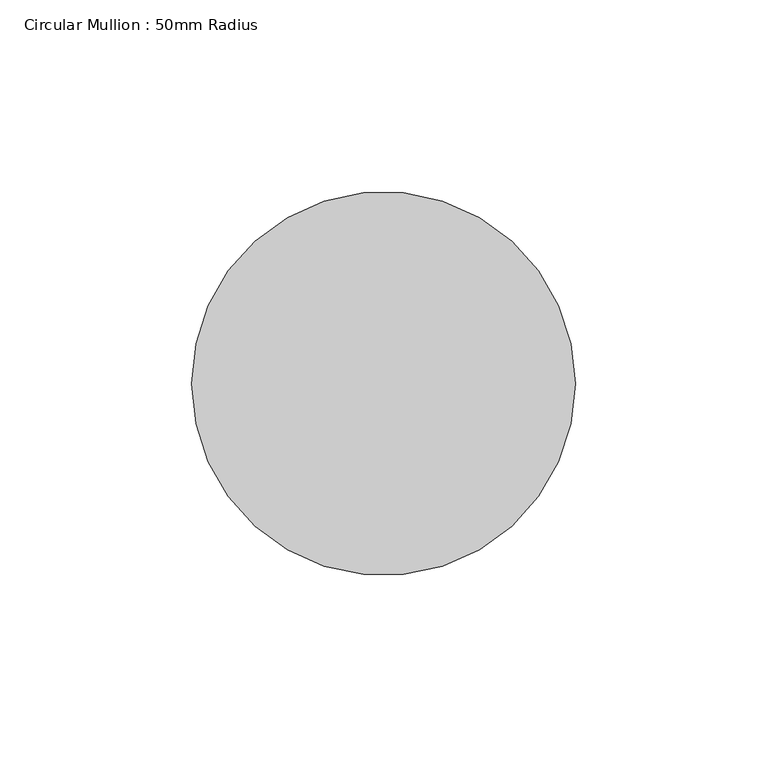
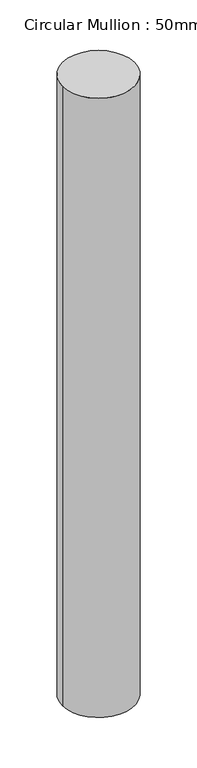
"""IFC4 building model written with IfcOpenShell, lengths in millimetres: member geometry, Circular Mullion : 50mm Radius."""

from ifc_helpers import new_model, si_unit, point, frame, origin, origin_2d, place, context, project, spatial, circle_curve, trimmed, segment, composite_curve, outline, extrude, source, transform, mapped, element, save


def circular_mullion_50mm_radius_90f196bb(model_context):
    return source(origin(), model_context, "Body", "SweptSolid", [
        extrude(outline(composite_curve([segment(trimmed(circle_curve(origin_2d(), 50.0), [point((50.0, 0.0))], [point((-50.0, 0.0))], False, "CARTESIAN"), True, "CONTINUOUS"), segment(trimmed(circle_curve(origin_2d(), 50.0), [point((-50.0, 0.0))], [point((50.0, 0.0))], False, "CARTESIAN"), True, "CONTINUOUS")], self_intersect=False)), frame((0.0, 0.0, -906.1521717), z_axis=(0.0, 0.0, 1.0), x_axis=(1.0, 0.0, 0.0)), (0.0, 0.0, 1.0), 906.1521717),
    ])


if __name__ == "__main__":
    model = new_model("IFC4")
    model_context = context("Model", 3, world=origin())
    ifc_project = project(units=[si_unit("LENGTHUNIT", "METRE", prefix="MILLI")], contexts=[model_context])
    site = spatial("IfcSite", under=ifc_project)
    building = spatial("IfcBuilding", under=site)
    placement = place(None, origin())
    circular_mullion_50mm_radius_shape = circular_mullion_50mm_radius_90f196bb(model_context)
    element("IfcMember", 1, ObjectType="Circular Mullion : 50mm Radius", at=placement, inside=building, context=model_context, shape_type="MappedRepresentation", body=[
        mapped(circular_mullion_50mm_radius_shape, transform((0.0, 0.0, 0.0), x_axis=(1.0, 0.0, 0.0), y_axis=(0.0, 1.0, 0.0), z_axis=(0.0, 0.0, 1.0))),
    ])
    save(model, "model.ifc")

# Revit data of these elements
# Type "Circular Mullion : 50mm Radius"
#   built-in parameter 1007350 = 0.164042 (stored number, unit not read)
# Element 1 (IfcMember, "Circular Mullion : 50mm Radius")
#   Materials on its faces: "Aluminium"
# Materials
#   "Aluminium": class "Metal", colour RGB 247 247 247, transparency 0, Description = "Aluminium 6061", Cost = 0
